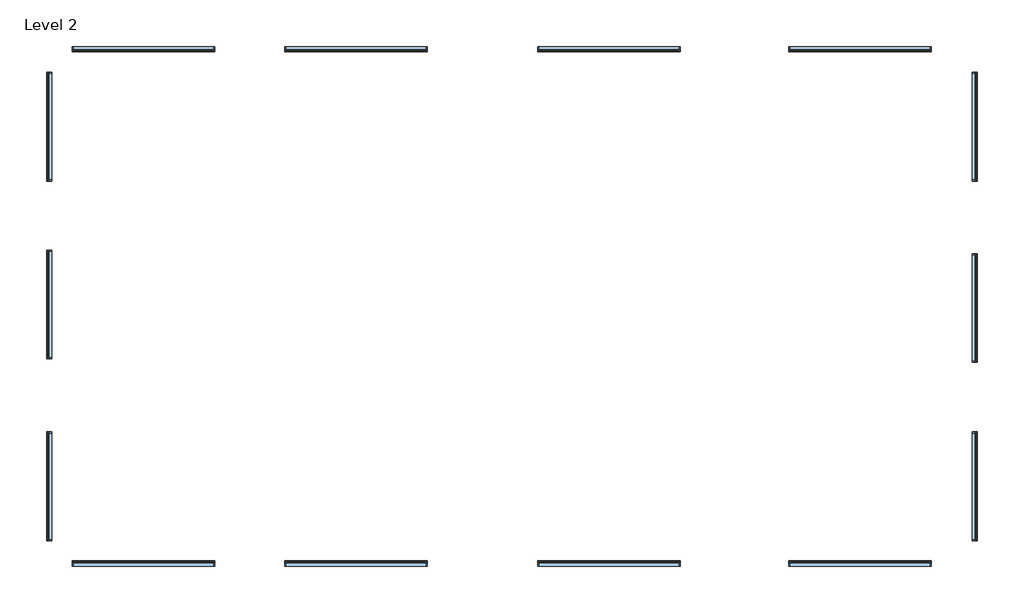
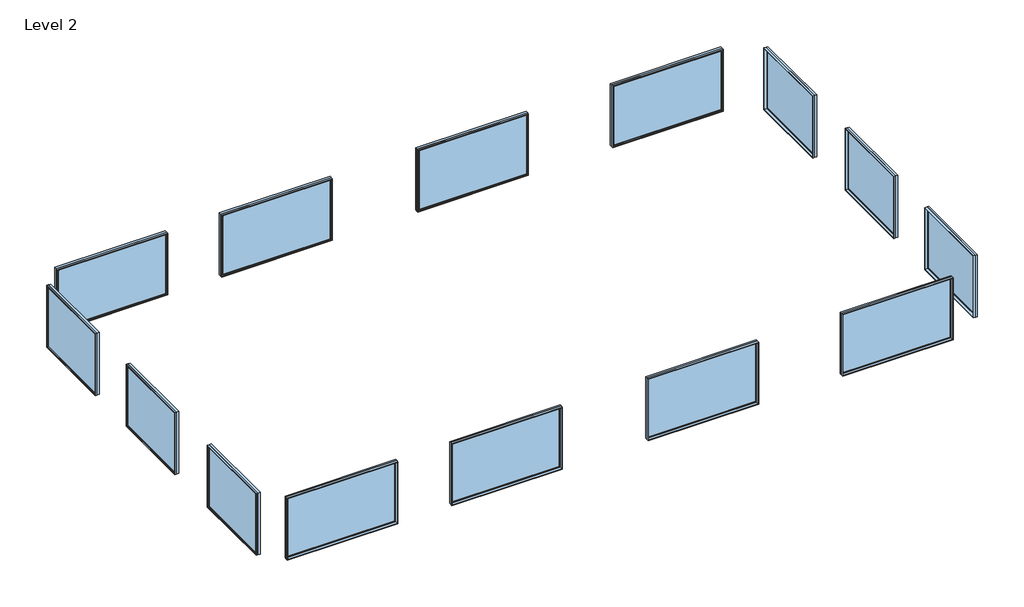
# One storey: 14 windows.
"""IFC4 building model written with IfcOpenShell, lengths in millimetres."""

import ifcopenshell
import ifcopenshell.guid

model = None  # the IFC model being written
_history = None  # IfcOwnerHistory: only IFC2X3 demands one
_inside = {}  # id of a spatial element -> (the spatial element, [elements in it])
_under = {}  # id of a project, library or spatial element -> (it, [spatial elements below it])
_declared = {}  # id of a project -> (the project, [libraries it declares])
_typed = {}  # id of a type object -> (the type object, [elements of that type])
_made_of = {}  # id of a material, layer set ... -> (it, [elements and type objects made of it])


def new_model(schema):
    """Start an empty IFC model of exactly this schema.

    Asked for "IFC4X3", IfcOpenShell would pick the latest addendum, in which some entities
    have other attributes; the version numbers below select the first issue.
    IFC2X3 requires an IfcOwnerHistory on every rooted entity: one is made here for all.
    """
    global model, _history
    if schema == "IFC4X3":
        model = ifcopenshell.file(schema_version=(4, 3, 0, 0))
    else:
        model = ifcopenshell.file(schema=schema)
    _inside.clear()
    _under.clear()
    _declared.clear()
    _typed.clear()
    _made_of.clear()
    _history = None
    if model.schema == "IFC2X3":
        org = make("IfcOrganization", Name="unknown")
        user = make(
            "IfcPersonAndOrganization",
            ThePerson=make("IfcPerson", FamilyName="unknown"),
            TheOrganization=org,
        )
        app = make(
            "IfcApplication",
            ApplicationDeveloper=org,
            Version="unknown",
            ApplicationFullName="unknown",
            ApplicationIdentifier="unknown",
        )
        _history = make(
            "IfcOwnerHistory",
            OwningUser=user,
            OwningApplication=app,
            ChangeAction="ADDED",
            CreationDate=0,
        )
    return model


def make(cls, **values):
    """One entity of the class cls with the attributes given. An attribute that is None is left unset."""
    return model.create_entity(
        cls, **{name: value for name, value in values.items() if value is not None}
    )


def rooted(cls, **values):
    """An entity with a GlobalId (a new one), such as an element, a storey or a relation."""
    return make(cls, GlobalId=ifcopenshell.guid.new(), OwnerHistory=_history, **values)


def si_unit(unit_type, name, prefix=None):
    """IfcSIUnit, for example si_unit("LENGTHUNIT", "METRE", prefix="MILLI")."""
    return make("IfcSIUnit", UnitType=unit_type, Prefix=prefix, Name=name)


def assignment(units):
    """IfcUnitAssignment: the units of a project."""
    return None if units is None else make("IfcUnitAssignment", Units=units)


def point(xyz):
    """IfcCartesianPoint."""
    return None if xyz is None else make("IfcCartesianPoint", Coordinates=xyz)


def direction(xyz):
    """IfcDirection."""
    return None if xyz is None else make("IfcDirection", DirectionRatios=xyz)


def frame(location, z_axis=None, x_axis=None):
    """IfcAxis2Placement3D, a coordinate frame: its origin and axes. An axis left out is left unset."""
    return make(
        "IfcAxis2Placement3D",
        Location=point(location),
        Axis=direction(z_axis),
        RefDirection=direction(x_axis),
    )


def origin():
    """The frame at (0, 0, 0) with its axes left unset."""
    return frame((0.0, 0.0, 0.0))


def place(relative_to, where):
    """IfcLocalPlacement: puts the frame where relative to a parent placement (None: the world)."""
    return make(
        "IfcLocalPlacement", PlacementRelTo=relative_to, RelativePlacement=where
    )


def context(
    kind, dimensions, precision=None, world=None, true_north=None, identifier=None
):
    """IfcGeometricRepresentationContext, for example the 3D "Model" context."""
    return make(
        "IfcGeometricRepresentationContext",
        ContextIdentifier=identifier,
        ContextType=kind,
        CoordinateSpaceDimension=dimensions,
        Precision=precision,
        WorldCoordinateSystem=world,
        TrueNorth=true_north,
    )


def project(units=None, contexts=None):
    """IfcProject with its units and contexts."""
    return rooted(
        "IfcProject",
        Name="project",
        RepresentationContexts=contexts,
        UnitsInContext=assignment(units),
    )


def spatial(cls, under=None, at=None, **own):
    """A site, building, storey or space (cls), placed at a placement, below another one or the project."""
    s = rooted(cls, ObjectPlacement=at, **own)
    if under is not None:
        _under.setdefault(under.id(), (under, []))[1].append(s)
    return s


def polyline(points):
    """IfcPolyline through the points."""
    return make("IfcPolyline", Points=[point(p) for p in points])


def outline(outer, holes=None, kind="AREA"):
    """IfcArbitraryClosedProfileDef: a profile drawn as a closed curve; with holes, ...WithVoids."""
    if holes is None:
        return make("IfcArbitraryClosedProfileDef", ProfileType=kind, OuterCurve=outer)
    return make(
        "IfcArbitraryProfileDefWithVoids",
        ProfileType=kind,
        OuterCurve=outer,
        InnerCurves=holes,
    )


def extrude(swept, where, along, depth):
    """IfcExtrudedAreaSolid: the profile swept, set in the frame where, extruded along a direction by depth."""
    return make(
        "IfcExtrudedAreaSolid",
        SweptArea=swept,
        Position=where,
        ExtrudedDirection=direction(along),
        Depth=depth,
    )


def shape(context_of_items, identifier, shape_type, items):
    """IfcShapeRepresentation: the items that make up one representation, for example the "Body"."""
    return make(
        "IfcShapeRepresentation",
        ContextOfItems=context_of_items,
        RepresentationIdentifier=identifier,
        RepresentationType=shape_type,
        Items=items,
    )


def source(mapping_origin, context_of_items, identifier, shape_type, items):
    """IfcRepresentationMap: a shape defined once, which mapped items show again and again."""
    return make(
        "IfcRepresentationMap",
        MappingOrigin=mapping_origin,
        MappedRepresentation=shape(context_of_items, identifier, shape_type, items),
    )


def transform(
    local_origin,
    x_axis=None,
    y_axis=None,
    z_axis=None,
    scale=None,
    scale2=None,
    scale3=None,
    uniform=True,
):
    """IfcCartesianTransformationOperator3D, or its non-uniform kind. x_axis, y_axis, z_axis: its Axis1, 2, 3."""
    if uniform:
        return make(
            "IfcCartesianTransformationOperator3D",
            Axis1=direction(x_axis),
            Axis2=direction(y_axis),
            LocalOrigin=point(local_origin),
            Scale=scale,
            Axis3=direction(z_axis),
        )
    return make(
        "IfcCartesianTransformationOperator3DnonUniform",
        Axis1=direction(x_axis),
        Axis2=direction(y_axis),
        LocalOrigin=point(local_origin),
        Scale=scale,
        Axis3=direction(z_axis),
        Scale2=scale2,
        Scale3=scale3,
    )


def mapped(mapping_source, mapping_target):
    """IfcMappedItem: shows the shape of a source again, moved by a transform."""
    return make(
        "IfcMappedItem", MappingSource=mapping_source, MappingTarget=mapping_target
    )


def made_of(thing, what):
    """Note that an element or type object is made of a material, layer set ...; save() writes the relation."""
    if what is not None:
        _made_of.setdefault(what.id(), (what, []))[1].append(thing)
    return thing


def element(
    cls,
    number,
    at=None,
    inside=None,
    cuts=None,
    type_object=None,
    material=None,
    context=None,
    identifier="Body",
    shape_type=None,
    held_by="IfcProductDefinitionShape",
    body=None,
    shapes=None,
    **own,
):
    """One element of the class cls, such as IfcWall. Its Tag is "e" and its number.

    at: its placement. inside: the storey or other place that contains it. cuts: it is an
    opening in that element (IfcRelVoidsElement). A single representation is given by context,
    identifier, shape_type and body (its items); several are given by shapes. held_by: the class
    of the entity that holds the representations. save() writes the other relations.
    """
    e = rooted(cls, Tag="e%d" % number, ObjectPlacement=at, **own)
    if body is not None:
        shapes = [shape(context, identifier, shape_type, body)]
    if shapes is not None:
        e.Representation = make(held_by, Representations=shapes)
    if inside is not None:
        _inside.setdefault(inside.id(), (inside, []))[1].append(e)
    if cuts is not None:
        rooted(
            "IfcRelVoidsElement", RelatingBuildingElement=cuts, RelatedOpeningElement=e
        )
    if type_object is not None:
        _typed.setdefault(type_object.id(), (type_object, []))[1].append(e)
    return made_of(e, material)


def aggregate(whole, parts):
    """IfcRelAggregates: a whole, such as a stair, and the parts it consists of."""
    return rooted("IfcRelAggregates", RelatingObject=whole, RelatedObjects=parts)


def save(model, path):
    """Write the relations noted so far, then the file.

    IfcRelAggregates (storeys below a building ...), IfcRelContainedInSpatialStructure (elements
    in a storey), IfcRelDefinesByType, IfcRelAssociatesMaterial and IfcRelDeclares: one each for
    every whole, place, type object, material and project.
    """
    for whole, parts in _under.values():
        aggregate(whole, parts)
    for where, things in _inside.values():
        rooted(
            "IfcRelContainedInSpatialStructure",
            RelatedElements=things,
            RelatingStructure=where,
        )
    for kind, things in _typed.values():
        rooted("IfcRelDefinesByType", RelatedObjects=things, RelatingType=kind)
    for what, things in _made_of.values():
        rooted("IfcRelAssociatesMaterial", RelatedObjects=things, RelatingMaterial=what)
    for by, libraries in _declared.values():
        rooted("IfcRelDeclares", RelatingContext=by, RelatedDefinitions=libraries)
    model.write(path)


def m_fixed_2500x_4228mm_fd5e51e7(model_context):
    return source(origin(), model_context, "Body", "SweptSolid", [
        extrude(outline(polyline([(-2050.8, 54.2), (2050.8, 54.2), (2050.8, 42.2), (-2050.8, 42.2), (-2050.8, 54.2)])), frame((0.0, 0.0, 368.0), z_axis=(0.0, 0.0, 1.0), x_axis=(1.0, 0.0, 0.0)), (0.0, 0.0, 1.0), 2374.0),
        extrude(outline(polyline([(2786.0, -2094.8), (324.0, -2094.8), (324.0, 2094.8), (2786.0, 2094.8), (2786.0, -2094.8)]), holes=[polyline([(2742.0, -2050.8), (2742.0, 2050.8), (368.0, 2050.8), (368.0, -2050.8), (2742.0, -2050.8)])]), frame((0.0, 26.2, 0.0), z_axis=(0.0, 1.0, 0.0), x_axis=(0.0, 0.0, 1.0)), (0.0, 0.0, 1.0), 44.0),
        extrude(outline(polyline([(2805.0, -2113.8), (305.0, -2113.8), (305.0, 2113.8), (2805.0, 2113.8), (2805.0, -2113.8)]), holes=[polyline([(2786.0, -2094.8), (2786.0, 2094.8), (324.0, 2094.8), (324.0, -2094.8), (2786.0, -2094.8)])]), frame((0.0, 26.2, 0.0), z_axis=(0.0, 1.0, 0.0), x_axis=(0.0, 0.0, 1.0)), (0.0, 0.0, 1.0), 63.0),
        extrude(outline(polyline([(2805.0, -2113.8), (305.0, -2113.8), (305.0, 2113.8), (2805.0, 2113.8), (2805.0, -2113.8)]), holes=[polyline([(2773.0, -2081.8), (2773.0, 2081.8), (337.0, 2081.8), (337.0, -2081.8), (2773.0, -2081.8)])]), frame((0.0, -63.2, 0.0), z_axis=(0.0, 1.0, 0.0), x_axis=(0.0, 0.0, 1.0)), (0.0, 0.0, 1.0), 89.4),
    ])


def m_fixed_2500x_4228mm_f14c179f(model_context):
    return source(origin(), model_context, "Body", "SweptSolid", [
        extrude(outline(polyline([(-2050.8, -54.2), (-2050.8, -42.2), (2050.8, -42.2), (2050.8, -54.2), (-2050.8, -54.2)])), frame((0.0, 0.0, 368.0), z_axis=(0.0, 0.0, 1.0), x_axis=(1.0, 0.0, 0.0)), (0.0, 0.0, 1.0), 2374.0),
        extrude(outline(polyline([(2786.0, -2094.8), (324.0, -2094.8), (324.0, 2094.8), (2786.0, 2094.8), (2786.0, -2094.8)]), holes=[polyline([(2742.0, -2050.8), (2742.0, 2050.8), (368.0, 2050.8), (368.0, -2050.8), (2742.0, -2050.8)])]), frame((0.0, -70.2, 0.0), z_axis=(0.0, 1.0, 0.0), x_axis=(0.0, 0.0, 1.0)), (0.0, 0.0, 1.0), 44.0),
        extrude(outline(polyline([(2805.0, -2113.8), (305.0, -2113.8), (305.0, 2113.8), (2805.0, 2113.8), (2805.0, -2113.8)]), holes=[polyline([(2786.0, -2094.8), (2786.0, 2094.8), (324.0, 2094.8), (324.0, -2094.8), (2786.0, -2094.8)])]), frame((0.0, -89.2, 0.0), z_axis=(0.0, 1.0, 0.0), x_axis=(0.0, 0.0, 1.0)), (0.0, 0.0, 1.0), 63.0),
        extrude(outline(polyline([(2805.0, -2113.8), (305.0, -2113.8), (305.0, 2113.8), (2805.0, 2113.8), (2805.0, -2113.8)]), holes=[polyline([(2773.0, -2081.8), (2773.0, 2081.8), (337.0, 2081.8), (337.0, -2081.8), (2773.0, -2081.8)])]), frame((0.0, -26.2, 0.0), z_axis=(0.0, 1.0, 0.0), x_axis=(0.0, 0.0, 1.0)), (0.0, 0.0, 1.0), 89.4),
    ])


def m_fixed_2500x_3220mm_df94f4d0(model_context):
    return source(origin(), model_context, "Body", "SweptSolid", [
        extrude(outline(polyline([(-1546.8, 54.2), (1546.8, 54.2), (1546.8, 42.2), (-1546.8, 42.2), (-1546.8, 54.2)])), frame((0.0, 0.0, 368.0), z_axis=(0.0, 0.0, 1.0), x_axis=(1.0, 0.0, 0.0)), (0.0, 0.0, 1.0), 2374.0),
        extrude(outline(polyline([(2786.0, -1590.8), (324.0, -1590.8), (324.0, 1590.8), (2786.0, 1590.8), (2786.0, -1590.8)]), holes=[polyline([(2742.0, -1546.8), (2742.0, 1546.8), (368.0, 1546.8), (368.0, -1546.8), (2742.0, -1546.8)])]), frame((0.0, 26.2, 0.0), z_axis=(0.0, 1.0, 0.0), x_axis=(0.0, 0.0, 1.0)), (0.0, 0.0, 1.0), 44.0),
        extrude(outline(polyline([(2805.0, -1609.8), (305.0, -1609.8), (305.0, 1609.8), (2805.0, 1609.8), (2805.0, -1609.8)]), holes=[polyline([(2786.0, -1590.8), (2786.0, 1590.8), (324.0, 1590.8), (324.0, -1590.8), (2786.0, -1590.8)])]), frame((0.0, 26.2, 0.0), z_axis=(0.0, 1.0, 0.0), x_axis=(0.0, 0.0, 1.0)), (0.0, 0.0, 1.0), 63.0),
        extrude(outline(polyline([(2805.0, -1609.8), (305.0, -1609.8), (305.0, 1609.8), (2805.0, 1609.8), (2805.0, -1609.8)]), holes=[polyline([(2773.0, -1577.8), (2773.0, 1577.8), (337.0, 1577.8), (337.0, -1577.8), (2773.0, -1577.8)])]), frame((0.0, -63.2, 0.0), z_axis=(0.0, 1.0, 0.0), x_axis=(0.0, 0.0, 1.0)), (0.0, 0.0, 1.0), 89.4),
    ])


def m_fixed_2500x_3220mm_8b997f8c(model_context):
    return source(origin(), model_context, "Body", "SweptSolid", [
        extrude(outline(polyline([(-1546.8, -54.2), (-1546.8, -42.2), (1546.8, -42.2), (1546.8, -54.2), (-1546.8, -54.2)])), frame((0.0, 0.0, 368.0), z_axis=(0.0, 0.0, 1.0), x_axis=(1.0, 0.0, 0.0)), (0.0, 0.0, 1.0), 2374.0),
        extrude(outline(polyline([(2786.0, -1590.8), (324.0, -1590.8), (324.0, 1590.8), (2786.0, 1590.8), (2786.0, -1590.8)]), holes=[polyline([(2742.0, -1546.8), (2742.0, 1546.8), (368.0, 1546.8), (368.0, -1546.8), (2742.0, -1546.8)])]), frame((0.0, -70.2, 0.0), z_axis=(0.0, 1.0, 0.0), x_axis=(0.0, 0.0, 1.0)), (0.0, 0.0, 1.0), 44.0),
        extrude(outline(polyline([(2805.0, -1609.8), (305.0, -1609.8), (305.0, 1609.8), (2805.0, 1609.8), (2805.0, -1609.8)]), holes=[polyline([(2786.0, -1590.8), (2786.0, 1590.8), (324.0, 1590.8), (324.0, -1590.8), (2786.0, -1590.8)])]), frame((0.0, -89.2, 0.0), z_axis=(0.0, 1.0, 0.0), x_axis=(0.0, 0.0, 1.0)), (0.0, 0.0, 1.0), 63.0),
        extrude(outline(polyline([(2805.0, -1609.8), (305.0, -1609.8), (305.0, 1609.8), (2805.0, 1609.8), (2805.0, -1609.8)]), holes=[polyline([(2773.0, -1577.8), (2773.0, 1577.8), (337.0, 1577.8), (337.0, -1577.8), (2773.0, -1577.8)])]), frame((0.0, -26.2, 0.0), z_axis=(0.0, 1.0, 0.0), x_axis=(0.0, 0.0, 1.0)), (0.0, 0.0, 1.0), 89.4),
    ])


model = new_model("IFC4")

# Units and contexts
model_context = context("Model", 3, world=origin())
ifc_project = project(units=[si_unit("LENGTHUNIT", "METRE", prefix="MILLI")], contexts=[model_context])

# Site, building, storey
site = spatial("IfcSite", under=ifc_project)
building = spatial("IfcBuilding", under=site)
storey = spatial("IfcBuildingStorey", under=building, Name="Level 2", Elevation=3962.4)

# Windows
placement = place(None, origin())
m_fixed_2500x_4228mm_shape = m_fixed_2500x_4228mm_fd5e51e7(model_context)
element("IfcWindow", 1, ObjectType="M_Fixed : 2500X 4228mm", at=placement, inside=storey, context=model_context, shape_type="MappedRepresentation", body=[
    mapped(m_fixed_2500x_4228mm_shape, transform((4360.264681, 11233.7802217, 4557.4), x_axis=(-1.0, 0.0, 0.0), y_axis=(0.0, -1.0, 0.0), z_axis=(0.0, 0.0, 1.0))),
])
element("IfcWindow", 2, ObjectType="M_Fixed : 2500X 4228mm", at=placement, inside=storey, context=model_context, shape_type="MappedRepresentation", body=[
    mapped(m_fixed_2500x_4228mm_shape, transform((10652.264681, 11233.7802217, 4557.4), x_axis=(-1.0, 0.0, 0.0), y_axis=(0.0, -1.0, 0.0), z_axis=(0.0, 0.0, 1.0))),
])
element("IfcWindow", 3, ObjectType="M_Fixed : 2500X 4228mm", at=placement, inside=storey, context=model_context, shape_type="MappedRepresentation", body=[
    mapped(m_fixed_2500x_4228mm_shape, transform((18152.264681, 11233.7802217, 4557.4), x_axis=(-1.0, 0.0, 0.0), y_axis=(0.0, -1.0, 0.0), z_axis=(0.0, 0.0, 1.0))),
])
element("IfcWindow", 4, ObjectType="M_Fixed : 2500X 4228mm", at=placement, inside=storey, context=model_context, shape_type="MappedRepresentation", body=[
    mapped(m_fixed_2500x_4228mm_shape, transform((25592.264681, 11233.7802217, 4557.4), x_axis=(-1.0, 0.0, 0.0), y_axis=(0.0, -1.0, 0.0), z_axis=(0.0, 0.0, 1.0))),
])
m_fixed_2500x_4228mm_2_shape = m_fixed_2500x_4228mm_f14c179f(model_context)
element("IfcWindow", 5, ObjectType="M_Fixed : 2500X 4228mm", at=placement, inside=storey, context=model_context, shape_type="MappedRepresentation", body=[
    mapped(m_fixed_2500x_4228mm_2_shape, transform((4360.264681, -4032.2197783, 4557.4), x_axis=(-1.0, 0.0, 0.0), y_axis=(0.0, -1.0, 0.0), z_axis=(0.0, 0.0, 1.0))),
])
element("IfcWindow", 6, ObjectType="M_Fixed : 2500X 4228mm", at=placement, inside=storey, context=model_context, shape_type="MappedRepresentation", body=[
    mapped(m_fixed_2500x_4228mm_2_shape, transform((10652.264681, -4032.2197783, 4557.4), x_axis=(-1.0, 0.0, 0.0), y_axis=(0.0, -1.0, 0.0), z_axis=(0.0, 0.0, 1.0))),
])
element("IfcWindow", 7, ObjectType="M_Fixed : 2500X 4228mm", at=placement, inside=storey, context=model_context, shape_type="MappedRepresentation", body=[
    mapped(m_fixed_2500x_4228mm_2_shape, transform((18152.264681, -4032.2197783, 4557.4), x_axis=(-1.0, 0.0, 0.0), y_axis=(0.0, -1.0, 0.0), z_axis=(0.0, 0.0, 1.0))),
])
element("IfcWindow", 8, ObjectType="M_Fixed : 2500X 4228mm", at=placement, inside=storey, context=model_context, shape_type="MappedRepresentation", body=[
    mapped(m_fixed_2500x_4228mm_2_shape, transform((25592.264681, -4032.2197783, 4557.4), x_axis=(-1.0, 0.0, 0.0), y_axis=(0.0, -1.0, 0.0), z_axis=(0.0, 0.0, 1.0))),
])
m_fixed_2500x_3220mm_shape = m_fixed_2500x_3220mm_df94f4d0(model_context)
element("IfcWindow", 9, ObjectType="M_Fixed : 2500x 3220mm", at=placement, inside=storey, context=model_context, shape_type="MappedRepresentation", body=[
    mapped(m_fixed_2500x_3220mm_shape, transform((1573.264681, 8920.7802217, 4559.8), x_axis=(0.0, 1.0, 0.0), y_axis=(-1.0, 0.0, 0.0), z_axis=(0.0, 0.0, 1.0))),
])
element("IfcWindow", 10, ObjectType="M_Fixed : 2500x 3220mm", at=placement, inside=storey, context=model_context, shape_type="MappedRepresentation", body=[
    mapped(m_fixed_2500x_3220mm_shape, transform((1573.264681, 3652.7802217, 4559.8), x_axis=(0.0, 1.0, 0.0), y_axis=(-1.0, 0.0, 0.0), z_axis=(0.0, 0.0, 1.0))),
])
element("IfcWindow", 11, ObjectType="M_Fixed : 2500x 3220mm", at=placement, inside=storey, context=model_context, shape_type="MappedRepresentation", body=[
    mapped(m_fixed_2500x_3220mm_shape, transform((1573.264681, -1733.2197783, 4559.8), x_axis=(0.0, 1.0, 0.0), y_axis=(-1.0, 0.0, 0.0), z_axis=(0.0, 0.0, 1.0))),
])
m_fixed_2500x_3220mm_2_shape = m_fixed_2500x_3220mm_8b997f8c(model_context)
element("IfcWindow", 12, ObjectType="M_Fixed : 2500x 3220mm", at=placement, inside=storey, context=model_context, shape_type="MappedRepresentation", body=[
    mapped(m_fixed_2500x_3220mm_2_shape, transform((28979.264681, 8920.7802217, 4559.8), x_axis=(0.0, 1.0, 0.0), y_axis=(-1.0, 0.0, 0.0), z_axis=(0.0, 0.0, 1.0))),
])
element("IfcWindow", 13, ObjectType="M_Fixed : 2500x 3220mm", at=placement, inside=storey, context=model_context, shape_type="MappedRepresentation", body=[
    mapped(m_fixed_2500x_3220mm_2_shape, transform((28979.264681, 3552.7802217, 4559.8), x_axis=(0.0, 1.0, 0.0), y_axis=(-1.0, 0.0, 0.0), z_axis=(0.0, 0.0, 1.0))),
])
element("IfcWindow", 14, ObjectType="M_Fixed : 2500x 3220mm", at=placement, inside=storey, context=model_context, shape_type="MappedRepresentation", body=[
    mapped(m_fixed_2500x_3220mm_2_shape, transform((28979.264681, -1733.2197783, 4559.8), x_axis=(0.0, 1.0, 0.0), y_axis=(-1.0, 0.0, 0.0), z_axis=(0.0, 0.0, 1.0))),
])

save(model, "model.ifc")

# Revit data of these elements
# Type "M_Fixed : 2500X 4228mm"
#   Type Mark = "25"
#   Height = 2500 mm
#   Default Sill Height = 305 mm
#   Width = 4227.6 mm
#   Window Inset = 19 mm
#   Frame Exterior Material = Sash
#   Frame Interior Material = Sash
#   Glass Pane Material = Glass
#   Sash = Sash
#   Wall Closure = (empty or 0)
# Type "M_Fixed : 2500x 3220mm"
#   Type Mark = "26"
#   Height = 2500 mm
#   Default Sill Height = 305 mm
#   Width = 3219.6 mm
#   Window Inset = 19 mm
#   Frame Exterior Material = Sash
#   Frame Interior Material = Sash
#   Glass Pane Material = Glass
#   Sash = Sash
#   Wall Closure = (empty or 0)
# Element 1 (IfcWindow, "M_Fixed : 2500X 4228mm")
#   Mark = "1"
#   Phase Created = New Construction
#   Materials on its faces: "Sash", "Glass"
# Element 2 (IfcWindow, "M_Fixed : 2500X 4228mm")
#   Mark = "2"
#   Phase Created = New Construction
#   Materials on its faces: "Sash", "Glass"
# Element 3 (IfcWindow, "M_Fixed : 2500X 4228mm")
#   Mark = "3"
#   Phase Created = New Construction
#   Materials on its faces: "Sash", "Glass"
# Element 4 (IfcWindow, "M_Fixed : 2500X 4228mm")
#   Mark = "4"
#   Phase Created = New Construction
#   Materials on its faces: "Sash", "Glass"
# Element 5 (IfcWindow, "M_Fixed : 2500X 4228mm")
#   Mark = "5"
#   Phase Created = New Construction
#   Materials on its faces: "Sash", "Glass"
# Element 6 (IfcWindow, "M_Fixed : 2500X 4228mm")
#   Mark = "6"
#   Phase Created = New Construction
#   Materials on its faces: "Sash", "Glass"
# Element 7 (IfcWindow, "M_Fixed : 2500X 4228mm")
#   Mark = "7"
#   Phase Created = New Construction
#   Materials on its faces: "Sash", "Glass"
# Element 8 (IfcWindow, "M_Fixed : 2500X 4228mm")
#   Mark = "8"
#   Phase Created = New Construction
#   Materials on its faces: "Sash", "Glass"
# Element 9 (IfcWindow, "M_Fixed : 2500x 3220mm")
#   Mark = "9"
#   Phase Created = New Construction
#   Materials on its faces: "Sash", "Glass"
# Element 10 (IfcWindow, "M_Fixed : 2500x 3220mm")
#   Mark = "18"
#   Phase Created = New Construction
#   Materials on its faces: "Sash", "Glass"
# Element 11 (IfcWindow, "M_Fixed : 2500x 3220mm")
#   Mark = "19"
#   Phase Created = New Construction
#   Materials on its faces: "Sash", "Glass"
# Element 12 (IfcWindow, "M_Fixed : 2500x 3220mm")
#   Mark = "20"
#   Phase Created = New Construction
#   Materials on its faces: "Sash", "Glass"
# Element 13 (IfcWindow, "M_Fixed : 2500x 3220mm")
#   Mark = "21"
#   Phase Created = New Construction
#   Materials on its faces: "Sash", "Glass"
# Element 14 (IfcWindow, "M_Fixed : 2500x 3220mm")
#   Mark = "22"
#   Phase Created = New Construction
#   Materials on its faces: "Sash", "Glass"
# Materials
#   "Sash": class "Wood", colour RGB 136 99 55, transparency 0
#   "Glass": class "Glass", colour RGB 0 128 192, transparency 0.9, Description = "Soda Lime Glass", Cost = 0
# Room at (7460.375, 2027.612) mm, phase "New Construction", upper level "Level 2", upper offset 3962.4 mm, lower offset 0 mm
#   Number = "12"
#   Name = "Room"
# Room at (7460.375, 8629.992) mm, phase "New Construction", upper level "Level 2", upper offset 3962.4 mm, lower offset 0 mm
#   Number = "13"
#   Name = "Room"
